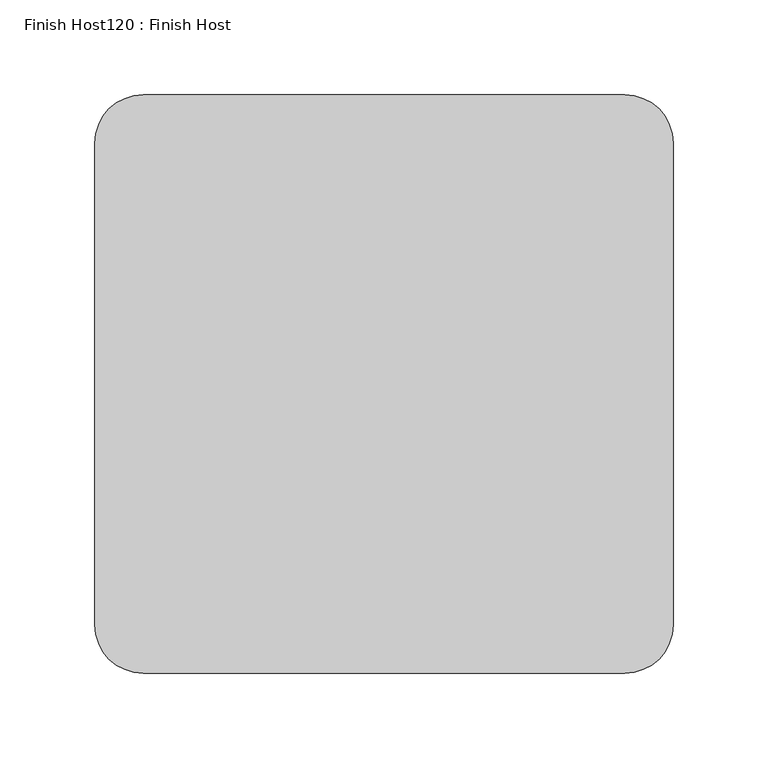
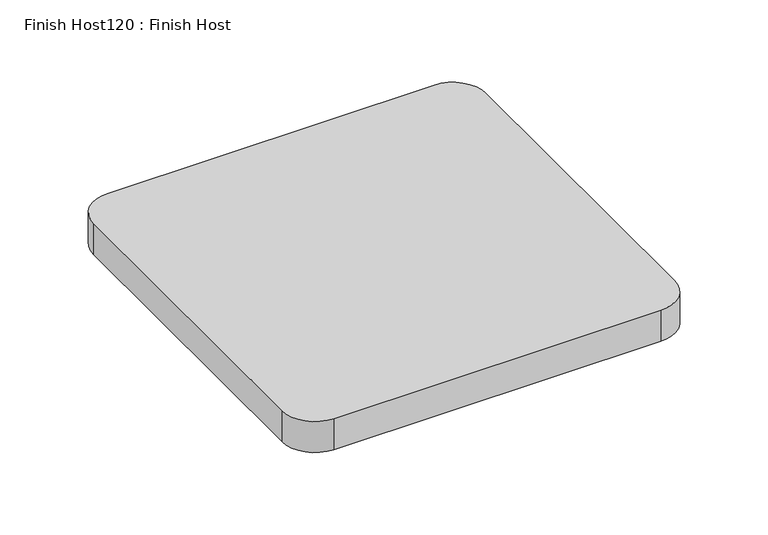
"""IFC4 building model written with IfcOpenShell, lengths in millimetres: proxy geometry, Finish Host120 : Finish Host."""

from ifc_helpers import new_model, si_unit, point, frame_2d, origin, origin_with_axes, place, context, project, spatial, polyline, circle_curve, trimmed, segment, composite_curve, outline, extrude, source, transform, mapped, element, save


def finish_host120_finish_host_94056946(model_context):
    return source(origin(), model_context, "Body", "SweptSolid", [
        extrude(outline(composite_curve([segment(polyline([(-797.1842816, 3462.3960864), (-797.1842816, 3716.3960864)]), True, "CONTINUOUS"), segment(trimmed(circle_curve(frame_2d((-771.7842816, 3716.3960864)), 25.4), [point((-797.1842816, 3716.3960864))], [point((-771.7842816, 3741.7960864))], False, "CARTESIAN"), True, "CONTINUOUS"), segment(polyline([(-771.7842816, 3741.7960864), (-517.7842816, 3741.7960864)]), True, "CONTINUOUS"), segment(trimmed(circle_curve(frame_2d((-517.7842816, 3716.3960864)), 25.4), [point((-517.7842816, 3741.7960864))], [point((-492.3842816, 3716.3960864))], False, "CARTESIAN"), True, "CONTINUOUS"), segment(polyline([(-492.3842816, 3716.3960864), (-492.3842816, 3462.3960864)]), True, "CONTINUOUS"), segment(trimmed(circle_curve(frame_2d((-517.7842816, 3462.3960864)), 25.4), [point((-492.3842816, 3462.3960864))], [point((-517.7842816, 3436.9960864))], False, "CARTESIAN"), True, "CONTINUOUS"), segment(polyline([(-517.7842816, 3436.9960864), (-771.7842816, 3436.9960864)]), True, "CONTINUOUS"), segment(trimmed(circle_curve(frame_2d((-771.7842816, 3462.3960864)), 25.4), [point((-771.7842816, 3436.9960864))], [point((-797.1842816, 3462.3960864))], False, "CARTESIAN"), True, "CONTINUOUS")], self_intersect=False)), origin_with_axes(), (0.0, 0.0, 1.0), 25.4),
    ])


if __name__ == "__main__":
    model = new_model("IFC4")
    model_context = context("Model", 3, world=origin())
    ifc_project = project(units=[si_unit("LENGTHUNIT", "METRE", prefix="MILLI")], contexts=[model_context])
    site = spatial("IfcSite", under=ifc_project)
    building = spatial("IfcBuilding", under=site)
    placement = place(None, origin())
    finish_host120_finish_host_shape = finish_host120_finish_host_94056946(model_context)
    element("IfcBuildingElementProxy", 1, Name="Finish Host120 : Finish Host", ObjectType="Finish Host120 : Finish Host", at=placement, inside=building, context=model_context, shape_type="MappedRepresentation", body=[
        mapped(finish_host120_finish_host_shape, transform((0.0, 0.0, 0.0), x_axis=(1.0, 0.0, 0.0), y_axis=(0.0, 1.0, 0.0), z_axis=(0.0, 0.0, 1.0))),
    ])
    save(model, "model.ifc")

# Revit data of these elements
# Type "Finish Host120 : Finish Host"
#   Panel Material = Fabric - Teknion - P113 - Percept - Tenet
# Element 1 (IfcBuildingElementProxy, "Finish Host120 : Finish Host")
#   Materials on its faces: "Fabric - Teknion - P113 - Percept - Tenet"
# Materials
#   "Fabric - Teknion - P113 - Percept - Tenet": class "Generic", colour RGB 79 96 94, transparency 0, Model = "P113", Manufacturer = "Teknion Textiles", URL = "http://www.tekniontextiles.ca/", Description = "Tenet Percept", Cost = 0
